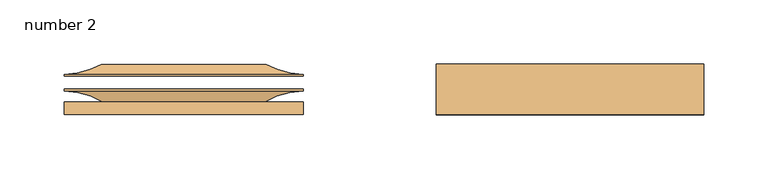
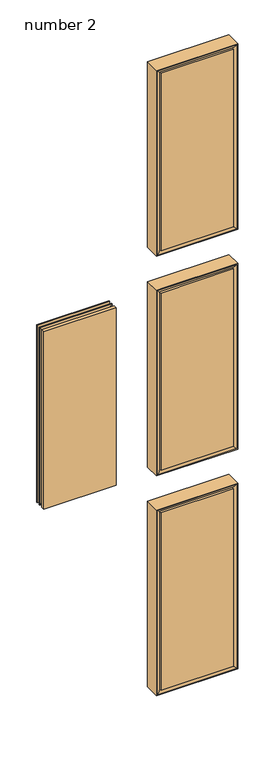
# IFC4 building model written with IfcOpenShell, lengths in millimetres: door geometry, Door-Interior-Karona-K5660-6_Panel : number 2.
# Revit data of these elements (continued)
# Type "Door-Interior-Karona-K5660-6_Panel : number 2" (continued)
#   Heat Transfer Coefficient (U) = 2.6120 W/(m²·K)
#   Daylight Opening Width = 0' - 0"
#   Daylight Opening Height = 0' - 0"
#   Bottom Rail Height = 0' - 8 1/2"
#   3D Open Angle = 0.00°
#   Thickness = 0' - 1 3/4"
#   Stop Thickness = 0' - 0 1/2"
#   Stop Depth = 0' - 1 3/8"
#   Rough Width = 2' - 7 29/32"
#   Rough Height = 6' - 8 61/64"
#   Rabbet Width = 0' - 1 3/4"
#   Jamb Offset = 0' - 0 61/64"
#   Hinge Offset = 0' - 0 3/4"
#   Jamb Thickness = 0' - 0 29/32"
#   Ext. Frame Thickness = 0' - 0 5/8"
#   Int. Frame Thickness = 0' - 0 5/8"
#   Height = 6' - 8"
#   Width = 2' - 6"
#   3D Angle = 0.00°
#   Trim Visible = yes
#   Square Sticking Profile = no
#   Raised Panel Door = yes
#   Ovolo Sticking Profile = yes
#   Ogee Sticking Profile = no
#   Mission Sticking Profile = no
#   Hinge Visible = yes
#   Glass Panel Door = no
#   Flat Panel Door = no
#   Edition number = 1
#   Define Thermal Properties by = 1
#   Trim Material = Wood - Karona - Red Oak
#   Top Rail Material = Wood - Karona - Red Oak
#   Stile Material = Wood - Karona - Red Oak
#   Sticking Material = Wood - Karona - Red Oak
#   Jamb Material = Wood - Karona - Red Oak
#   Interior Panel = Wood - Karona - Red Oak
#   Door Panel Material = Wood - Karona - Red Oak
#   Bottom Rail Material = Wood - Karona - Red Oak
#   Visual Light Transmittance = 0
#   Solar Heat Gain Coefficient = 0
#   Construction Type = (empty or 0)
#   Function = (empty or 0)
#   Wall Closure = (empty or 0)
# Element 1 (IfcDoor, "Door-Interior-Karona-K5660-6_Panel : number 2")
#   Materials on its faces: "Wood - Karona - Red Oak"
# Materials
#   "Wood - Karona - Red Oak": class "Wood", colour RGB 153 121 89, transparency 0, Description = "Quercus Rubra", Cost = 0
